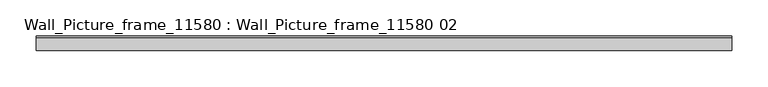
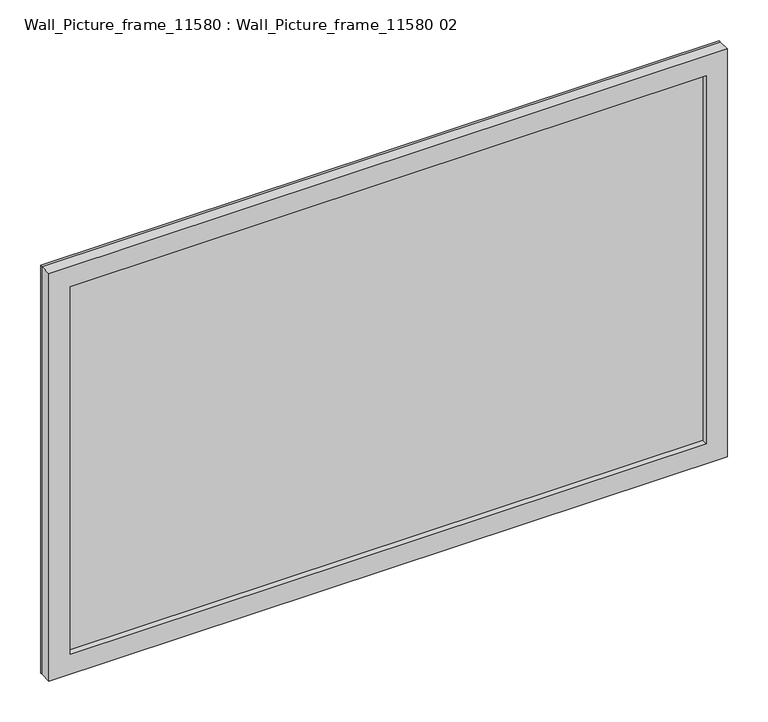
"""IFC4 building model written with IfcOpenShell, lengths in millimetres: furniture geometry, Wall_Picture_frame_11580 : Wall_Picture_frame_11580 02."""

from ifc_helpers import new_model, si_unit, frame, origin, origin_with_axes, place, context, project, spatial, polyline, outline, extrude, source, transform, mapped, element, save


def wall_picture_frame_11580_wall_picture_frame_11580_02_aef4a011(model_context):
    return source(origin(), model_context, "Body", "SweptSolid", [
        extrude(outline(polyline([(930.0, -12.0), (30.0, -12.0), (30.0, -10.0), (930.0, -10.0), (930.0, -12.0)])), frame((0.0, 0.0, 30.0), z_axis=(0.0, 0.0, 1.0), x_axis=(1.0, 0.0, 0.0)), (0.0, 0.0, 1.0), 550.0),
        extrude(outline(polyline([(855.0, -5.0), (105.0, -5.0), (105.0, -3.0), (855.0, -3.0), (855.0, -5.0)])), frame((0.0, 0.0, 105.0), z_axis=(0.0, 0.0, 1.0), x_axis=(1.0, 0.0, 0.0)), (0.0, 0.0, 1.0), 400.0),
        extrude(outline(polyline([(580.0, 930.0), (580.0, 30.0), (30.0, 30.0), (30.0, 930.0), (580.0, 930.0)]), holes=[polyline([(505.0, 855.0), (105.0, 855.0), (105.0, 105.0), (505.0, 105.0), (505.0, 855.0)])]), frame((0.0, -9.0, 0.0), z_axis=(0.0, 1.0, 0.0), x_axis=(0.0, 0.0, 1.0)), (0.0, 0.0, 1.0), 6.0),
        extrude(outline(polyline([(610.0, 0.0), (0.0, 0.0), (0.0, 960.0), (610.0, 960.0), (610.0, 0.0)]), holes=[polyline([(580.0, 930.0), (30.0, 930.0), (30.0, 30.0), (580.0, 30.0), (580.0, 930.0)])]), frame((0.0, -20.0, 0.0), z_axis=(0.0, 1.0, 0.0), x_axis=(0.0, 0.0, 1.0)), (0.0, 0.0, 1.0), 17.0),
        extrude(outline(polyline([(960.0, -3.0), (0.0, -3.0), (0.0, 0.0), (960.0, 0.0), (960.0, -3.0)])), origin_with_axes(), (0.0, 0.0, 1.0), 610.0),
    ])


if __name__ == "__main__":
    model = new_model("IFC4")
    model_context = context("Model", 3, world=origin())
    ifc_project = project(units=[si_unit("LENGTHUNIT", "METRE", prefix="MILLI")], contexts=[model_context])
    site = spatial("IfcSite", under=ifc_project)
    building = spatial("IfcBuilding", under=site)
    placement = place(None, origin())
    wall_picture_frame_11580_wall_picture_frame_11580_02_shape = wall_picture_frame_11580_wall_picture_frame_11580_02_aef4a011(model_context)
    element("IfcFurniture", 1, ObjectType="Wall_Picture_frame_11580 : Wall_Picture_frame_11580 02", at=placement, inside=building, context=model_context, shape_type="MappedRepresentation", body=[
        mapped(wall_picture_frame_11580_wall_picture_frame_11580_02_shape, transform((0.0, 0.0, 0.0), x_axis=(1.0, 0.0, 0.0), y_axis=(0.0, 1.0, 0.0), z_axis=(0.0, 0.0, 1.0))),
    ])
    save(model, "model.ifc")

# Revit data of these elements
# Type "Wall_Picture_frame_11580 : Wall_Picture_frame_11580 02"
#   Width [instance default] = 960 mm
#   Picture width [instance default] = 750 mm
#   Picture height [instance default] = 400 mm
#   Passepartout width [instance default] = 75 mm
#   Height [instance default] = 610 mm
#   Frame width [instance default] = 30 mm
#   Picture [instance default] = none
#   Passe-partout = Picture-Passepartout
#   Front glass = Picture-front glass
#   Frame = Picture-frame
# Element 1 (IfcFurniture, "Wall_Picture_frame_11580 : Wall_Picture_frame_11580 02")
#   Materials on its faces: "Picture-frame", "Picture-Passepartout", "Picture-front glass"
# Materials
#   "Picture-Passepartout": class "Miscellaneous", colour RGB 127 127 127, transparency 0
#   "Picture-front glass": class "Glass", colour RGB 250 250 250, transparency 0.9
#   "Picture-frame": class "Miscellaneous", colour RGB 3 3 3, transparency 0
